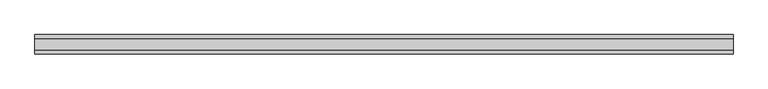
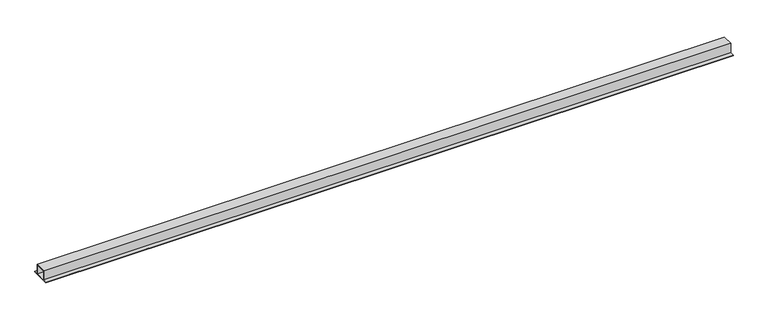
"""IFC4 building model written with IfcOpenShell, lengths in millimetres: beam geometry, NLRS_28_SF_LIB_stalen ligger THQ-AV-CWV-MMBS-SRP_gen_rsf : stalen ligger_gen__THQ_280x10-290x30-550x20."""

from ifc_helpers import new_model, si_unit, frame, origin, place, context, project, spatial, polyline, outline, extrude, source, transform, mapped, element, save


def beam_1759c74d(model_context):
    return source(origin(), model_context, "Body", "SweptSolid", [
        extrude(outline(polyline([(143.5, 280.0), (143.5, 0.0), (263.5, 0.0), (263.5, -20.0), (-286.5, -20.0), (-286.5, 0.0), (-166.5, 0.0), (-166.5, 280.0), (143.5, 280.0)]), holes=[polyline([(133.5, 0.0), (133.5, 250.0), (-156.5, 250.0), (-156.5, 0.0), (133.5, 0.0)])]), frame((-9887.5, 0.0, 0.0), z_axis=(1.0, 0.0, 0.0), x_axis=(0.0, 1.0, 0.0)), (0.0, 0.0, 1.0), 19775.0),
    ])


if __name__ == "__main__":
    model = new_model("IFC4")
    model_context = context("Model", 3, world=origin())
    ifc_project = project(units=[si_unit("LENGTHUNIT", "METRE", prefix="MILLI")], contexts=[model_context])
    site = spatial("IfcSite", under=ifc_project)
    building = spatial("IfcBuilding", under=site)
    placement = place(None, origin())
    beam_shape = beam_1759c74d(model_context)
    element("IfcBeam", 1, ObjectType="NLRS_28_SF_LIB_stalen ligger THQ-AV-CWV-MMBS-SRP_gen_rsf : stalen ligger_gen__THQ_280x10-290x30-550x20", at=placement, inside=building, context=model_context, shape_type="MappedRepresentation", body=[
        mapped(beam_shape, transform((0.0, 0.0, 0.0), x_axis=(1.0, 0.0, 0.0), y_axis=(0.0, 1.0, 0.0), z_axis=(0.0, 0.0, 1.0))),
    ])
    save(model, "model.ifc")

# Revit data of these elements
# Type "NLRS_28_SF_LIB_stalen ligger THQ-AV-CWV-MMBS-SRP_gen_rsf : stalen ligger_gen__THQ_280x10-290x30-550x20"
#   Type IfcGUID = "2GRbcre991teoKeCLB8MAm"
#   IfcExportAs = "IfcBeamType"
#   Type Comments = "THQ 280x10-290x30-550x20"
#   Model = " "
#   Manufacturer = " "
#   Fire Rating = " "
#   Description = "stalen ligger THQ 280x10-290x30-550x20"
#   Assembly Code = "28.11"
#   tw = 10 mm
#   tu = 20 mm
#   to = 30 mm
#   h = 280 mm
#   bu = 550 mm
#   bo = 290 mm
#   NLRS_C_lengte [instance default] = 1500 mm
#   Length [instance default] = 1500 mm
#   RSF_C_vullen_met_beton [instance default] = no
#   RSF_C_petligger = no
#   RSF_C_hoedligger = yes
#   Structural Material = NLRS_h2_staal_gen_rsf
#   Keynote = ""
# Element 1 (IfcBeam, "NLRS_28_SF_LIB_stalen ligger THQ-AV-CWV-MMBS-SRP_gen_rsf : stalen ligger_gen__THQ_280x10-290x30-550x20")
#   NLRS_C_lengte = 19775 mm
#   Materials on its faces: "NLRS_h2_staal_gen_rsf"
# Materials
#   "NLRS_h2_staal_gen_rsf": class "H - Metaal", colour RGB 189 187 185, transparency 0, Keynote = "h2", Manufacturer = "Revit Standards Foundation", URL = "www.revitstandards.org", Description = "staal", Cost = 0
